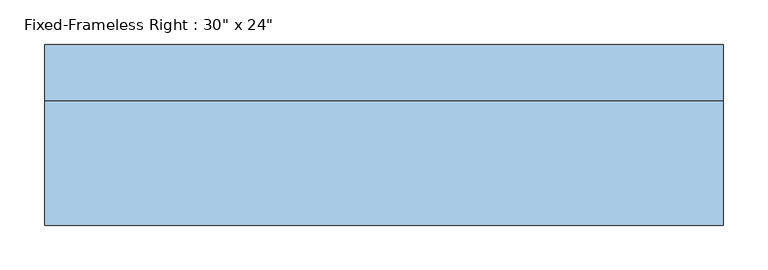
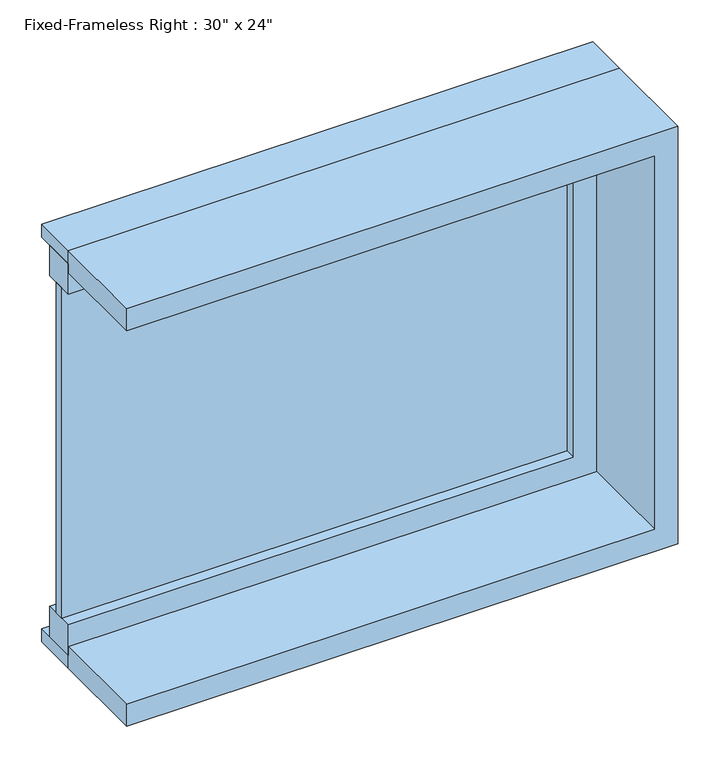
"""IFC4 building model written with IfcOpenShell, lengths in millimetres: window geometry."""

import ifcopenshell
import ifcopenshell.guid

model = None  # the IFC model being written
_history = None  # IfcOwnerHistory: only IFC2X3 demands one
_inside = {}  # id of a spatial element -> (the spatial element, [elements in it])
_under = {}  # id of a project, library or spatial element -> (it, [spatial elements below it])
_declared = {}  # id of a project -> (the project, [libraries it declares])
_typed = {}  # id of a type object -> (the type object, [elements of that type])
_made_of = {}  # id of a material, layer set ... -> (it, [elements and type objects made of it])


def new_model(schema):
    """Start an empty IFC model of exactly this schema.

    Asked for "IFC4X3", IfcOpenShell would pick the latest addendum, in which some entities
    have other attributes; the version numbers below select the first issue.
    IFC2X3 requires an IfcOwnerHistory on every rooted entity: one is made here for all.
    """
    global model, _history
    if schema == "IFC4X3":
        model = ifcopenshell.file(schema_version=(4, 3, 0, 0))
    else:
        model = ifcopenshell.file(schema=schema)
    _inside.clear()
    _under.clear()
    _declared.clear()
    _typed.clear()
    _made_of.clear()
    _history = None
    if model.schema == "IFC2X3":
        org = make("IfcOrganization", Name="unknown")
        user = make(
            "IfcPersonAndOrganization",
            ThePerson=make("IfcPerson", FamilyName="unknown"),
            TheOrganization=org,
        )
        app = make(
            "IfcApplication",
            ApplicationDeveloper=org,
            Version="unknown",
            ApplicationFullName="unknown",
            ApplicationIdentifier="unknown",
        )
        _history = make(
            "IfcOwnerHistory",
            OwningUser=user,
            OwningApplication=app,
            ChangeAction="ADDED",
            CreationDate=0,
        )
    return model


def make(cls, **values):
    """One entity of the class cls with the attributes given. An attribute that is None is left unset."""
    return model.create_entity(
        cls, **{name: value for name, value in values.items() if value is not None}
    )


def rooted(cls, **values):
    """An entity with a GlobalId (a new one), such as an element, a storey or a relation."""
    return make(cls, GlobalId=ifcopenshell.guid.new(), OwnerHistory=_history, **values)


def si_unit(unit_type, name, prefix=None):
    """IfcSIUnit, for example si_unit("LENGTHUNIT", "METRE", prefix="MILLI")."""
    return make("IfcSIUnit", UnitType=unit_type, Prefix=prefix, Name=name)


def assignment(units):
    """IfcUnitAssignment: the units of a project."""
    return None if units is None else make("IfcUnitAssignment", Units=units)


def point(xyz):
    """IfcCartesianPoint."""
    return None if xyz is None else make("IfcCartesianPoint", Coordinates=xyz)


def direction(xyz):
    """IfcDirection."""
    return None if xyz is None else make("IfcDirection", DirectionRatios=xyz)


def frame(location, z_axis=None, x_axis=None):
    """IfcAxis2Placement3D, a coordinate frame: its origin and axes. An axis left out is left unset."""
    return make(
        "IfcAxis2Placement3D",
        Location=point(location),
        Axis=direction(z_axis),
        RefDirection=direction(x_axis),
    )


def origin():
    """The frame at (0, 0, 0) with its axes left unset."""
    return frame((0.0, 0.0, 0.0))


def place(relative_to, where):
    """IfcLocalPlacement: puts the frame where relative to a parent placement (None: the world)."""
    return make(
        "IfcLocalPlacement", PlacementRelTo=relative_to, RelativePlacement=where
    )


def context(
    kind, dimensions, precision=None, world=None, true_north=None, identifier=None
):
    """IfcGeometricRepresentationContext, for example the 3D "Model" context."""
    return make(
        "IfcGeometricRepresentationContext",
        ContextIdentifier=identifier,
        ContextType=kind,
        CoordinateSpaceDimension=dimensions,
        Precision=precision,
        WorldCoordinateSystem=world,
        TrueNorth=true_north,
    )


def project(units=None, contexts=None):
    """IfcProject with its units and contexts."""
    return rooted(
        "IfcProject",
        Name="project",
        RepresentationContexts=contexts,
        UnitsInContext=assignment(units),
    )


def spatial(cls, under=None, at=None, **own):
    """A site, building, storey or space (cls), placed at a placement, below another one or the project."""
    s = rooted(cls, ObjectPlacement=at, **own)
    if under is not None:
        _under.setdefault(under.id(), (under, []))[1].append(s)
    return s


def polyline(points):
    """IfcPolyline through the points."""
    return make("IfcPolyline", Points=[point(p) for p in points])


def outline(outer, holes=None, kind="AREA"):
    """IfcArbitraryClosedProfileDef: a profile drawn as a closed curve; with holes, ...WithVoids."""
    if holes is None:
        return make("IfcArbitraryClosedProfileDef", ProfileType=kind, OuterCurve=outer)
    return make(
        "IfcArbitraryProfileDefWithVoids",
        ProfileType=kind,
        OuterCurve=outer,
        InnerCurves=holes,
    )


def extrude(swept, where, along, depth):
    """IfcExtrudedAreaSolid: the profile swept, set in the frame where, extruded along a direction by depth."""
    return make(
        "IfcExtrudedAreaSolid",
        SweptArea=swept,
        Position=where,
        ExtrudedDirection=direction(along),
        Depth=depth,
    )


def shape(context_of_items, identifier, shape_type, items):
    """IfcShapeRepresentation: the items that make up one representation, for example the "Body"."""
    return make(
        "IfcShapeRepresentation",
        ContextOfItems=context_of_items,
        RepresentationIdentifier=identifier,
        RepresentationType=shape_type,
        Items=items,
    )


def source(mapping_origin, context_of_items, identifier, shape_type, items):
    """IfcRepresentationMap: a shape defined once, which mapped items show again and again."""
    return make(
        "IfcRepresentationMap",
        MappingOrigin=mapping_origin,
        MappedRepresentation=shape(context_of_items, identifier, shape_type, items),
    )


def transform(
    local_origin,
    x_axis=None,
    y_axis=None,
    z_axis=None,
    scale=None,
    scale2=None,
    scale3=None,
    uniform=True,
):
    """IfcCartesianTransformationOperator3D, or its non-uniform kind. x_axis, y_axis, z_axis: its Axis1, 2, 3."""
    if uniform:
        return make(
            "IfcCartesianTransformationOperator3D",
            Axis1=direction(x_axis),
            Axis2=direction(y_axis),
            LocalOrigin=point(local_origin),
            Scale=scale,
            Axis3=direction(z_axis),
        )
    return make(
        "IfcCartesianTransformationOperator3DnonUniform",
        Axis1=direction(x_axis),
        Axis2=direction(y_axis),
        LocalOrigin=point(local_origin),
        Scale=scale,
        Axis3=direction(z_axis),
        Scale2=scale2,
        Scale3=scale3,
    )


def mapped(mapping_source, mapping_target):
    """IfcMappedItem: shows the shape of a source again, moved by a transform."""
    return make(
        "IfcMappedItem", MappingSource=mapping_source, MappingTarget=mapping_target
    )


def made_of(thing, what):
    """Note that an element or type object is made of a material, layer set ...; save() writes the relation."""
    if what is not None:
        _made_of.setdefault(what.id(), (what, []))[1].append(thing)
    return thing


def element(
    cls,
    number,
    at=None,
    inside=None,
    cuts=None,
    type_object=None,
    material=None,
    context=None,
    identifier="Body",
    shape_type=None,
    held_by="IfcProductDefinitionShape",
    body=None,
    shapes=None,
    **own,
):
    """One element of the class cls, such as IfcWall. Its Tag is "e" and its number.

    at: its placement. inside: the storey or other place that contains it. cuts: it is an
    opening in that element (IfcRelVoidsElement). A single representation is given by context,
    identifier, shape_type and body (its items); several are given by shapes. held_by: the class
    of the entity that holds the representations. save() writes the other relations.
    """
    e = rooted(cls, Tag="e%d" % number, ObjectPlacement=at, **own)
    if body is not None:
        shapes = [shape(context, identifier, shape_type, body)]
    if shapes is not None:
        e.Representation = make(held_by, Representations=shapes)
    if inside is not None:
        _inside.setdefault(inside.id(), (inside, []))[1].append(e)
    if cuts is not None:
        rooted(
            "IfcRelVoidsElement", RelatingBuildingElement=cuts, RelatedOpeningElement=e
        )
    if type_object is not None:
        _typed.setdefault(type_object.id(), (type_object, []))[1].append(e)
    return made_of(e, material)


def aggregate(whole, parts):
    """IfcRelAggregates: a whole, such as a stair, and the parts it consists of."""
    return rooted("IfcRelAggregates", RelatingObject=whole, RelatedObjects=parts)


def save(model, path):
    """Write the relations noted so far, then the file.

    IfcRelAggregates (storeys below a building ...), IfcRelContainedInSpatialStructure (elements
    in a storey), IfcRelDefinesByType, IfcRelAssociatesMaterial and IfcRelDeclares: one each for
    every whole, place, type object, material and project.
    """
    for whole, parts in _under.values():
        aggregate(whole, parts)
    for where, things in _inside.values():
        rooted(
            "IfcRelContainedInSpatialStructure",
            RelatedElements=things,
            RelatingStructure=where,
        )
    for kind, things in _typed.values():
        rooted("IfcRelDefinesByType", RelatedObjects=things, RelatingType=kind)
    for what, things in _made_of.values():
        rooted("IfcRelAssociatesMaterial", RelatedObjects=things, RelatingMaterial=what)
    for by, libraries in _declared.values():
        rooted("IfcRelDeclares", RelatingContext=by, RelatedDefinitions=libraries)
    model.write(path)


def window_e8819a91(model_context):
    return source(origin(), model_context, "Body", "SweptSolid", [
        extrude(outline(polyline([(279.4, 53.975), (-419.1, 53.975), (-419.1, 66.675), (279.4, 66.675), (279.4, 53.975)])), frame((0.0, 0.0, 977.9), z_axis=(0.0, 0.0, 1.0), x_axis=(1.0, 0.0, 0.0)), (0.0, 0.0, 1.0), 482.6),
        extrude(outline(polyline([(1504.95, -419.1), (1460.5, -419.1), (1460.5, 279.4), (977.9, 279.4), (977.9, -419.1), (933.45, -419.1), (933.45, 323.85), (1504.95, 323.85), (1504.95, -419.1)])), frame((0.0, 38.1, 0.0), z_axis=(0.0, 1.0, 0.0), x_axis=(0.0, 0.0, 1.0)), (0.0, 0.0, 1.0), 44.45),
        extrude(outline(polyline([(1524.0, -419.1), (1492.25, -419.1), (1492.25, 311.15), (946.15, 311.15), (946.15, -419.1), (914.4, -419.1), (914.4, 342.9), (1524.0, 342.9), (1524.0, -419.1)])), frame((0.0, -101.6, 0.0), z_axis=(0.0, 1.0, 0.0), x_axis=(0.0, 0.0, 1.0)), (0.0, 0.0, 1.0), 139.7),
        extrude(outline(polyline([(1524.0, 342.9), (1524.0, -419.1), (1504.95, -419.1), (1504.95, 323.85), (933.45, 323.85), (933.45, -419.1), (914.4, -419.1), (914.4, 342.9), (1524.0, 342.9)])), frame((0.0, 38.1, 0.0), z_axis=(0.0, 1.0, 0.0), x_axis=(0.0, 0.0, 1.0)), (0.0, 0.0, 1.0), 63.5),
    ])


if __name__ == "__main__":
    model = new_model("IFC4")
    model_context = context("Model", 3, world=origin())
    ifc_project = project(units=[si_unit("LENGTHUNIT", "METRE", prefix="MILLI")], contexts=[model_context])
    site = spatial("IfcSite", under=ifc_project)
    building = spatial("IfcBuilding", under=site)
    placement = place(None, origin())
    window_shape = window_e8819a91(model_context)
    element("IfcWindow", 1, ObjectType="Fixed-Frameless Right : 30\" x 24\"", at=placement, inside=building, context=model_context, shape_type="MappedRepresentation", body=[
        mapped(window_shape, transform((0.0, 0.0, 0.0), x_axis=(1.0, 0.0, 0.0), y_axis=(0.0, 1.0, 0.0), z_axis=(0.0, 0.0, 1.0))),
    ])
    save(model, "model.ifc")

# Revit data of these elements
# Type "Fixed-Frameless Right : 30\" x 24\""
#   Type Mark = "78"
#   Assembly Code = "B2020100"
#   Height = 609.60 mm
#   Default Sill Height = 914.40 mm
#   Width = 762.00 mm
#   Window Inset = 19.05 mm
#   Glass Pane Material = Glass
#   Sash Material = Sash
#   Wall Closure = (empty or 0)
# Element 1 (IfcWindow, "Fixed-Frameless Right : 30\" x 24\"")
#   Materials on its faces: "Sash", "Glass"
# Materials
#   "Glass": class "Glass", colour RGB 0 128 192, transparency 0.75
#   "Sash": class "Wood", colour RGB 224 178 126, transparency 0
